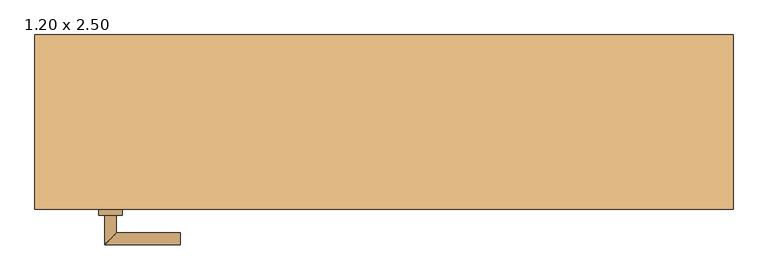
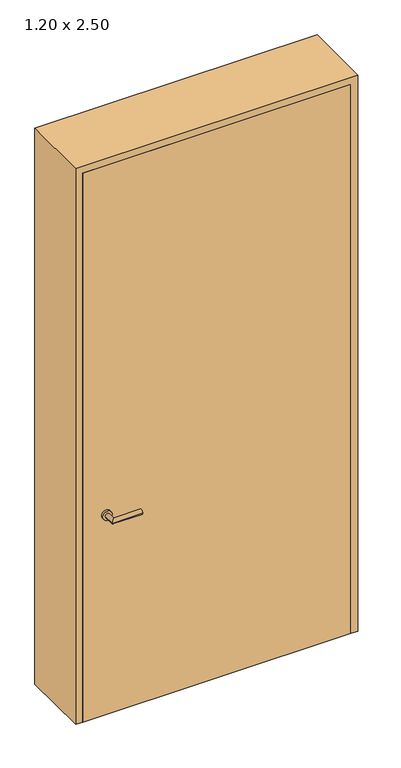
"""IFC4 building model written with IfcOpenShell, lengths in millimetres: door geometry, Drehflügel 1-flg - Blockzarge : 1.20 x 2.50."""

from ifc_helpers import new_model, si_unit, point, frame, frame_2d, origin, place, context, project, spatial, polyline, circle_curve, ellipse_curve, trimmed, segment, composite_curve, outline, extrude, source, transform, mapped, element, save
from ifc_brep_helpers import plane_surface, cylinder_surface, advanced_brep


def door_1_20_x_2_50_96f548bd(model_context):
    return source(origin(), model_context, "Body", "SolidModel", [
        advanced_brep(
        [(-460.0, -129.4346141, 1000.0), (-480.0, -129.4346141, 1000.0), (-480.0, -79.4346141, 1000.0), (-460.0, -99.4346141, 1000.0), (-350.0, -99.4346141, 1000.0), (-350.0, -79.4346141, 1000.0)],
        [
            (0, 1, circle_curve(frame((-470.0, -129.4346141, 1000.0), z_axis=(0.0, -1.0, 0.0), x_axis=(-1.0, 0.0, 0.0)), 10.0)),
            (1, 0, circle_curve(frame((-470.0, -129.4346141, 1000.0), z_axis=(0.0, -1.0, 0.0), x_axis=(-1.0, 0.0, 0.0)), 10.0)),
            (1, 2),
            (2, 3, ellipse_curve(frame((-470.0, -89.4346141, 1000.0), z_axis=(-0.7071067811865686, -0.7071067811865265, 0.0), x_axis=(0.7071067811865264, -0.7071067811865687, 0.0)), 14.1421356, 10.0)),
            (3, 0),
            (3, 2, ellipse_curve(frame((-470.0, -89.4346141, 1000.0), z_axis=(-0.7071067811865686, -0.7071067811865265, 0.0), x_axis=(0.7071067811865264, -0.7071067811865687, 0.0)), 14.1421356, 10.0)),
            (4, 5, circle_curve(frame((-350.0, -89.4346141, 1000.0), z_axis=(1.0, 0.0, 0.0), x_axis=(0.0, 1.0, 0.0)), 10.0)),
            (5, 4, circle_curve(frame((-350.0, -89.4346141, 1000.0), z_axis=(1.0, 0.0, 0.0), x_axis=(0.0, 1.0, 0.0)), 10.0)),
            (2, 5),
            (4, 3),
        ],
        [
            plane_surface(frame((-470.0, -129.4346141, -287.7526403), z_axis=(0.0, -1.0, 0.0), x_axis=(0.0, 0.0, 1.0))),
            cylinder_surface(frame((-470.0, -129.4346141, 1000.0), z_axis=(0.0, -1.0, 0.0), x_axis=(-1.0, 0.0, 0.0)), 10.0),
            plane_surface(frame((-350.0, -89.4346141, -287.7526403), z_axis=(1.0, 0.0, 0.0), x_axis=(0.0, 0.0, 1.0))),
            cylinder_surface(frame((-470.0, -89.4346141, 1000.0), z_axis=(-1.0, 0.0, 0.0), x_axis=(0.0, 1.0, 0.0)), 10.0),
        ],
        [
            (0, [[1, 2]]),
            (1, [[3, 4, 5, -2]]),
            (1, [[-5, 6, -3, -1]]),
            (2, [[7, 8]]),
            (3, [[9, -7, 10, -4]]),
            (3, [[-10, -8, -9, -6]]),
        ],
    ),
        advanced_brep(
        [(-460.0, -174.4346141, 1000.0), (-480.0, -174.4346141, 1000.0), (-480.0, -224.4346141, 1000.0), (-460.0, -204.4346141, 1000.0), (-350.0, -204.4346141, 1000.0), (-350.0, -224.4346141, 1000.0)],
        [
            (0, 1, circle_curve(frame((-470.0, -174.4346141, 1000.0), z_axis=(0.0, 1.0, 0.0), x_axis=(-1.0, 0.0, 0.0)), 10.0)),
            (1, 0, circle_curve(frame((-470.0, -174.4346141, 1000.0), z_axis=(0.0, 1.0, 0.0), x_axis=(-1.0, 0.0, 0.0)), 10.0)),
            (1, 2),
            (2, 3, ellipse_curve(frame((-470.0, -214.4346141, 1000.0), z_axis=(-0.7071067811865486, 0.7071067811865464, 0.0), x_axis=(0.7071067811865464, 0.7071067811865488, 0.0)), 14.1421356, 10.0)),
            (3, 0),
            (3, 2, ellipse_curve(frame((-470.0, -214.4346141, 1000.0), z_axis=(-0.7071067811865486, 0.7071067811865464, 0.0), x_axis=(0.7071067811865464, 0.7071067811865488, 0.0)), 14.1421356, 10.0)),
            (4, 5, circle_curve(frame((-350.0, -214.4346141, 1000.0), z_axis=(1.0, 0.0, 0.0), x_axis=(0.0, -1.0, 0.0)), 10.0)),
            (5, 4, circle_curve(frame((-350.0, -214.4346141, 1000.0), z_axis=(1.0, 0.0, 0.0), x_axis=(0.0, -1.0, 0.0)), 10.0)),
            (2, 5),
            (4, 3),
        ],
        [
            plane_surface(frame((-470.0, -174.4346141, -287.7526403), z_axis=(0.0, 1.0, 0.0), x_axis=(0.0, 0.0, 1.0))),
            cylinder_surface(frame((-470.0, -174.4346141, 1000.0), z_axis=(0.0, 1.0, 0.0), x_axis=(-1.0, 0.0, 0.0)), 10.0),
            plane_surface(frame((-350.0, -214.4346141, -287.7526403), z_axis=(1.0, 0.0, 0.0), x_axis=(0.0, 0.0, 1.0))),
            cylinder_surface(frame((-470.0, -214.4346141, 1000.0), z_axis=(-1.0, 0.0, 0.0), x_axis=(0.0, -1.0, 0.0)), 10.0),
        ],
        [
            (0, [[1, 2]]),
            (1, [[3, 4, 5, -2]]),
            (1, [[-5, 6, -3, -1]]),
            (2, [[7, 8]]),
            (3, [[9, -7, 10, -4]]),
            (3, [[-10, -8, -9, -6]]),
        ],
    ),
        extrude(outline(composite_curve([segment(trimmed(circle_curve(frame_2d((1000.0, -470.0)), 20.0), [point((1000.0, -450.0))], [point((1000.0, -490.0))], False, "CARTESIAN"), True, "CONTINUOUS"), segment(trimmed(circle_curve(frame_2d((1000.0, -470.0)), 20.0), [point((1000.0, -490.0))], [point((1000.0, -450.0))], False, "CARTESIAN"), True, "CONTINUOUS")], self_intersect=False)), frame((0.0, -139.4346141, 0.0), z_axis=(0.0, 1.0, 0.0), x_axis=(0.0, 0.0, 1.0)), (0.0, 0.0, 1.0), 10.0),
        extrude(outline(composite_curve([segment(trimmed(circle_curve(frame_2d((1000.0, -470.0)), 20.0), [point((1000.0, -450.0))], [point((1000.0, -490.0))], False, "CARTESIAN"), True, "CONTINUOUS"), segment(trimmed(circle_curve(frame_2d((1000.0, -470.0)), 20.0), [point((1000.0, -490.0))], [point((1000.0, -450.0))], False, "CARTESIAN"), True, "CONTINUOUS")], self_intersect=False)), frame((0.0, -174.4346141, 0.0), z_axis=(0.0, 1.0, 0.0), x_axis=(0.0, 0.0, 1.0)), (0.0, 0.0, 1.0), 10.0),
        extrude(outline(polyline([(2600.0, 600.0), (2600.0, -600.0), (100.0, -600.0), (100.0, -570.0), (2570.0, -570.0), (2570.0, 570.0), (100.0, 570.0), (100.0, 600.0), (2600.0, 600.0)])), frame((0.0, -164.4346141, 0.0), z_axis=(0.0, 1.0, 0.0), x_axis=(0.0, 0.0, 1.0)), (0.0, 0.0, 1.0), 300.0),
        extrude(outline(polyline([(570.0, -164.4346141), (-570.0, -164.4346141), (-570.0, -139.4346141), (570.0, -139.4346141), (570.0, -164.4346141)])), frame((0.0, 0.0, 100.0), z_axis=(0.0, 0.0, 1.0), x_axis=(1.0, 0.0, 0.0)), (0.0, 0.0, 1.0), 2470.0),
    ])


if __name__ == "__main__":
    model = new_model("IFC4")
    model_context = context("Model", 3, world=origin())
    ifc_project = project(units=[si_unit("LENGTHUNIT", "METRE", prefix="MILLI")], contexts=[model_context])
    site = spatial("IfcSite", under=ifc_project)
    building = spatial("IfcBuilding", under=site)
    placement = place(None, origin())
    door_1_20_x_2_50_shape = door_1_20_x_2_50_96f548bd(model_context)
    element("IfcDoor", 1, ObjectType="Drehflügel 1-flg - Blockzarge : 1.20 x 2.50", at=placement, inside=building, context=model_context, shape_type="MappedRepresentation", body=[
        mapped(door_1_20_x_2_50_shape, transform((0.0, 0.0, 0.0), x_axis=(1.0, 0.0, 0.0), y_axis=(0.0, 1.0, 0.0), z_axis=(0.0, 0.0, 1.0))),
    ])
    save(model, "model.ifc")

# Revit data of these elements
# Type "Drehflügel 1-flg - Blockzarge : 1.20 x 2.50"
#   Type Mark = "27"
#   Operation = "SingleSwingRight"
#   Keynote = "16.03"
#   Visual Light Transmittance = 0.9
#   Solar Heat Gain Coefficient = 0.86
#   Heat Transfer Coefficient (U) = 5.5617 W/(m²·K)
#   Rough Width = 1.200 m
#   Stärke Futter = 0.030 m
#   Rough Height [instance default] = 2.600 m
#   Höhe Türgriff = 0.900 m
#   Height = 2.500 m
#   Fußbodenaufbau [instance default] = 0.100 m
#   Width = 1.200 m
#   Sichtbarkeit Sturzlinien [instance default] = yes
#   Türgriff auswählen [instance default] = element 420047
#   Türgriff [instance default] = none
#   Türflügel [instance default] = none
#   Rahmen/Pfosten [instance default] = none
#   Construction Type Id = ""
#   Function = (empty or 0)
#   Wall Closure = (empty or 0)
#   Analytic Construction = (empty or 0)
# Element 1 (IfcDoor, "Drehflügel 1-flg - Blockzarge : 1.20 x 2.50")
#   Materials on its faces: "Metall - Chrom", "Holz - Birke"
# Materials
#   "Metall - Chrom": class "Metall", colour RGB 247 247 247, transparency 0, Cost = 0
#   "Holz - Birke": class "Holz", colour RGB 213 164 103, transparency 0, Cost = 0
